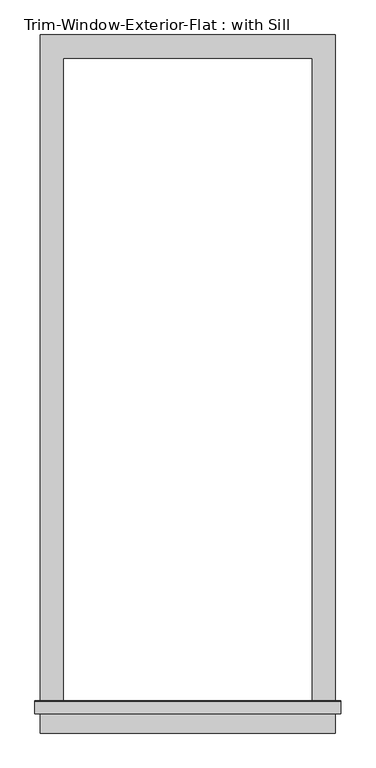
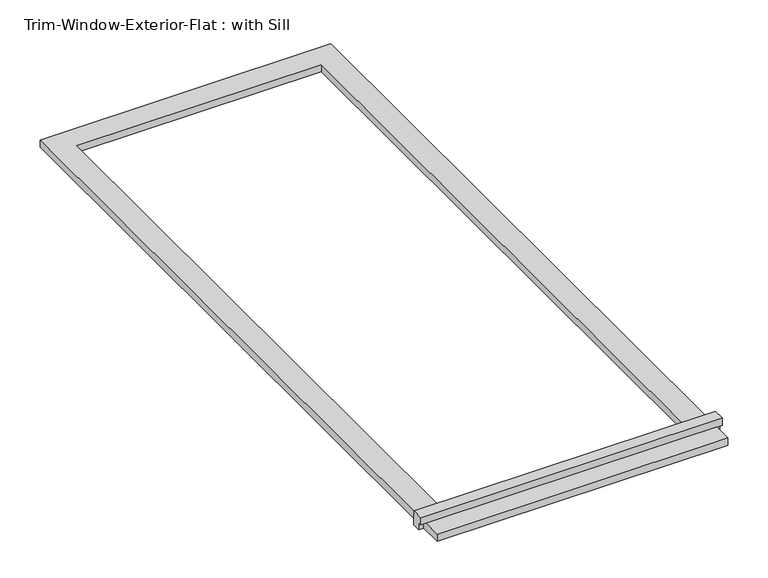
"""IFC4 building model written with IfcOpenShell, lengths in millimetres: proxy geometry, Trim-Window-Exterior-Flat : with Sill."""

from ifc_helpers import new_model, si_unit, frame, origin, origin_with_axes, place, context, project, spatial, polyline, outline, extrude, source, transform, mapped, element, save


def trim_window_exterior_flat_with_sill_acac9a23(model_context):
    return source(origin(), model_context, "Body", "SweptSolid", [
        extrude(outline(polyline([(361.95, -1596.9823709), (361.95, -1654.1323709), (-361.95, -1654.1323709), (-361.95, -1596.9823709), (361.95, -1596.9823709)])), origin_with_axes(), (0.0, 0.0, 1.0), 19.05),
        extrude(outline(polyline([(-1606.55, 38.1), (-1577.2580645, 38.1), (-1574.8, 19.05), (-1574.8, 0.0), (-1596.9823709, 0.0), (-1596.9823709, 19.05), (-1606.55, 19.05), (-1606.55, 38.1)])), frame((-374.65, 0.0, 0.0), z_axis=(1.0, 0.0, 0.0), x_axis=(0.0, 1.0, 0.0)), (0.0, 0.0, 1.0), 749.3),
        extrude(outline(polyline([(-361.95, 57.15), (361.95, 57.15), (361.95, -1574.8), (304.8, -1574.8), (304.8, 0.0), (-304.8, 0.0), (-304.8, -1574.8), (-361.95, -1574.8), (-361.95, 57.15)])), origin_with_axes(), (0.0, 0.0, 1.0), 19.05),
    ])


if __name__ == "__main__":
    model = new_model("IFC4")
    model_context = context("Model", 3, world=origin())
    ifc_project = project(units=[si_unit("LENGTHUNIT", "METRE", prefix="MILLI")], contexts=[model_context])
    site = spatial("IfcSite", under=ifc_project)
    building = spatial("IfcBuilding", under=site)
    placement = place(None, origin())
    trim_window_exterior_flat_with_sill_shape = trim_window_exterior_flat_with_sill_acac9a23(model_context)
    element("IfcBuildingElementProxy", 1, Name="Trim-Window-Exterior-Flat : with Sill", ObjectType="Trim-Window-Exterior-Flat : with Sill", at=placement, inside=building, context=model_context, shape_type="MappedRepresentation", body=[
        mapped(trim_window_exterior_flat_with_sill_shape, transform((0.0, 0.0, 0.0), x_axis=(1.0, 0.0, 0.0), y_axis=(0.0, 1.0, 0.0), z_axis=(0.0, 0.0, 1.0))),
    ])
    save(model, "model.ifc")

# Revit data of these elements
# Type "Trim-Window-Exterior-Flat : with Sill"
#   Trim Width = 0' - 2 1/4"
#   Trim Thickness_Picture Frame = 0' - 1 1/4"
#   Trim Thickness_with Sill = 0' - 0 3/4"
#   Sill Thickness = 0' - 1 1/4"
#   Opening Width [instance default] = 2' - 0"
#   Opening Height [instance default] = 3' - 0"
#   Default Elevation = 4' - 0"
#   Sill = yes
#   Picture Frame = no
#   Trim Material [instance default] = none
# Element 1 (IfcBuildingElementProxy, "Trim-Window-Exterior-Flat : with Sill")
#   Opening Height = 5' - 2"
#   Trim Material = Clad - White
#   Materials on its faces: "Clad - White"
# Materials
#   "Clad - White": class "Wood", colour RGB 245 245 243, transparency 0, Cost = 0
